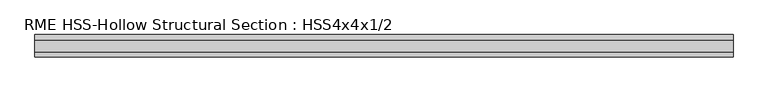
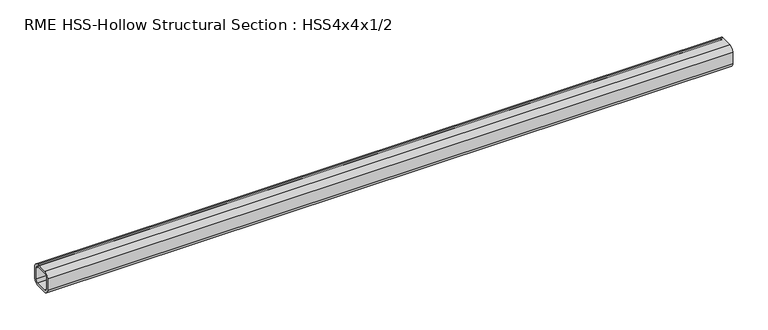
"""IFC4 building model written with IfcOpenShell, lengths in millimetres: member geometry, RME HSS-Hollow Structural Section : HSS4x4x1/2."""

import ifcopenshell
import ifcopenshell.guid

model = None  # the IFC model being written
_history = None  # IfcOwnerHistory: only IFC2X3 demands one
_inside = {}  # id of a spatial element -> (the spatial element, [elements in it])
_under = {}  # id of a project, library or spatial element -> (it, [spatial elements below it])
_declared = {}  # id of a project -> (the project, [libraries it declares])
_typed = {}  # id of a type object -> (the type object, [elements of that type])
_made_of = {}  # id of a material, layer set ... -> (it, [elements and type objects made of it])


def new_model(schema):
    """Start an empty IFC model of exactly this schema.

    Asked for "IFC4X3", IfcOpenShell would pick the latest addendum, in which some entities
    have other attributes; the version numbers below select the first issue.
    IFC2X3 requires an IfcOwnerHistory on every rooted entity: one is made here for all.
    """
    global model, _history
    if schema == "IFC4X3":
        model = ifcopenshell.file(schema_version=(4, 3, 0, 0))
    else:
        model = ifcopenshell.file(schema=schema)
    _inside.clear()
    _under.clear()
    _declared.clear()
    _typed.clear()
    _made_of.clear()
    _history = None
    if model.schema == "IFC2X3":
        org = make("IfcOrganization", Name="unknown")
        user = make(
            "IfcPersonAndOrganization",
            ThePerson=make("IfcPerson", FamilyName="unknown"),
            TheOrganization=org,
        )
        app = make(
            "IfcApplication",
            ApplicationDeveloper=org,
            Version="unknown",
            ApplicationFullName="unknown",
            ApplicationIdentifier="unknown",
        )
        _history = make(
            "IfcOwnerHistory",
            OwningUser=user,
            OwningApplication=app,
            ChangeAction="ADDED",
            CreationDate=0,
        )
    return model


def make(cls, **values):
    """One entity of the class cls with the attributes given. An attribute that is None is left unset."""
    return model.create_entity(
        cls, **{name: value for name, value in values.items() if value is not None}
    )


def rooted(cls, **values):
    """An entity with a GlobalId (a new one), such as an element, a storey or a relation."""
    return make(cls, GlobalId=ifcopenshell.guid.new(), OwnerHistory=_history, **values)


def si_unit(unit_type, name, prefix=None):
    """IfcSIUnit, for example si_unit("LENGTHUNIT", "METRE", prefix="MILLI")."""
    return make("IfcSIUnit", UnitType=unit_type, Prefix=prefix, Name=name)


def assignment(units):
    """IfcUnitAssignment: the units of a project."""
    return None if units is None else make("IfcUnitAssignment", Units=units)


def point(xyz):
    """IfcCartesianPoint."""
    return None if xyz is None else make("IfcCartesianPoint", Coordinates=xyz)


def direction(xyz):
    """IfcDirection."""
    return None if xyz is None else make("IfcDirection", DirectionRatios=xyz)


def frame(location, z_axis=None, x_axis=None):
    """IfcAxis2Placement3D, a coordinate frame: its origin and axes. An axis left out is left unset."""
    return make(
        "IfcAxis2Placement3D",
        Location=point(location),
        Axis=direction(z_axis),
        RefDirection=direction(x_axis),
    )


def frame_2d(location, x_axis=None):
    """IfcAxis2Placement2D, a coordinate frame in the plane: its origin and x axis."""
    return make(
        "IfcAxis2Placement2D", Location=point(location), RefDirection=direction(x_axis)
    )


def origin():
    """The frame at (0, 0, 0) with its axes left unset."""
    return frame((0.0, 0.0, 0.0))


def place(relative_to, where):
    """IfcLocalPlacement: puts the frame where relative to a parent placement (None: the world)."""
    return make(
        "IfcLocalPlacement", PlacementRelTo=relative_to, RelativePlacement=where
    )


def context(
    kind, dimensions, precision=None, world=None, true_north=None, identifier=None
):
    """IfcGeometricRepresentationContext, for example the 3D "Model" context."""
    return make(
        "IfcGeometricRepresentationContext",
        ContextIdentifier=identifier,
        ContextType=kind,
        CoordinateSpaceDimension=dimensions,
        Precision=precision,
        WorldCoordinateSystem=world,
        TrueNorth=true_north,
    )


def project(units=None, contexts=None):
    """IfcProject with its units and contexts."""
    return rooted(
        "IfcProject",
        Name="project",
        RepresentationContexts=contexts,
        UnitsInContext=assignment(units),
    )


def spatial(cls, under=None, at=None, **own):
    """A site, building, storey or space (cls), placed at a placement, below another one or the project."""
    s = rooted(cls, ObjectPlacement=at, **own)
    if under is not None:
        _under.setdefault(under.id(), (under, []))[1].append(s)
    return s


def polyline(points):
    """IfcPolyline through the points."""
    return make("IfcPolyline", Points=[point(p) for p in points])


def circle_curve(where, radius):
    """IfcCircle in the frame where."""
    return make("IfcCircle", Position=where, Radius=radius)


def trimmed(basis, trim1, trim2, sense, master):
    """IfcTrimmedCurve: the piece of a basis curve between two trims."""
    return make(
        "IfcTrimmedCurve",
        BasisCurve=basis,
        Trim1=trim1,
        Trim2=trim2,
        SenseAgreement=sense,
        MasterRepresentation=master,
    )


def segment(curve, same_sense, transition):
    """IfcCompositeCurveSegment."""
    return make(
        "IfcCompositeCurveSegment",
        Transition=transition,
        SameSense=same_sense,
        ParentCurve=curve,
    )


def composite_curve(segments, self_intersect=None):
    """IfcCompositeCurve: segments joined end to end."""
    return make("IfcCompositeCurve", Segments=segments, SelfIntersect=self_intersect)


def outline(outer, holes=None, kind="AREA"):
    """IfcArbitraryClosedProfileDef: a profile drawn as a closed curve; with holes, ...WithVoids."""
    if holes is None:
        return make("IfcArbitraryClosedProfileDef", ProfileType=kind, OuterCurve=outer)
    return make(
        "IfcArbitraryProfileDefWithVoids",
        ProfileType=kind,
        OuterCurve=outer,
        InnerCurves=holes,
    )


def extrude(swept, where, along, depth):
    """IfcExtrudedAreaSolid: the profile swept, set in the frame where, extruded along a direction by depth."""
    return make(
        "IfcExtrudedAreaSolid",
        SweptArea=swept,
        Position=where,
        ExtrudedDirection=direction(along),
        Depth=depth,
    )


def shape(context_of_items, identifier, shape_type, items):
    """IfcShapeRepresentation: the items that make up one representation, for example the "Body"."""
    return make(
        "IfcShapeRepresentation",
        ContextOfItems=context_of_items,
        RepresentationIdentifier=identifier,
        RepresentationType=shape_type,
        Items=items,
    )


def source(mapping_origin, context_of_items, identifier, shape_type, items):
    """IfcRepresentationMap: a shape defined once, which mapped items show again and again."""
    return make(
        "IfcRepresentationMap",
        MappingOrigin=mapping_origin,
        MappedRepresentation=shape(context_of_items, identifier, shape_type, items),
    )


def transform(
    local_origin,
    x_axis=None,
    y_axis=None,
    z_axis=None,
    scale=None,
    scale2=None,
    scale3=None,
    uniform=True,
):
    """IfcCartesianTransformationOperator3D, or its non-uniform kind. x_axis, y_axis, z_axis: its Axis1, 2, 3."""
    if uniform:
        return make(
            "IfcCartesianTransformationOperator3D",
            Axis1=direction(x_axis),
            Axis2=direction(y_axis),
            LocalOrigin=point(local_origin),
            Scale=scale,
            Axis3=direction(z_axis),
        )
    return make(
        "IfcCartesianTransformationOperator3DnonUniform",
        Axis1=direction(x_axis),
        Axis2=direction(y_axis),
        LocalOrigin=point(local_origin),
        Scale=scale,
        Axis3=direction(z_axis),
        Scale2=scale2,
        Scale3=scale3,
    )


def mapped(mapping_source, mapping_target):
    """IfcMappedItem: shows the shape of a source again, moved by a transform."""
    return make(
        "IfcMappedItem", MappingSource=mapping_source, MappingTarget=mapping_target
    )


def made_of(thing, what):
    """Note that an element or type object is made of a material, layer set ...; save() writes the relation."""
    if what is not None:
        _made_of.setdefault(what.id(), (what, []))[1].append(thing)
    return thing


def element(
    cls,
    number,
    at=None,
    inside=None,
    cuts=None,
    type_object=None,
    material=None,
    context=None,
    identifier="Body",
    shape_type=None,
    held_by="IfcProductDefinitionShape",
    body=None,
    shapes=None,
    **own,
):
    """One element of the class cls, such as IfcWall. Its Tag is "e" and its number.

    at: its placement. inside: the storey or other place that contains it. cuts: it is an
    opening in that element (IfcRelVoidsElement). A single representation is given by context,
    identifier, shape_type and body (its items); several are given by shapes. held_by: the class
    of the entity that holds the representations. save() writes the other relations.
    """
    e = rooted(cls, Tag="e%d" % number, ObjectPlacement=at, **own)
    if body is not None:
        shapes = [shape(context, identifier, shape_type, body)]
    if shapes is not None:
        e.Representation = make(held_by, Representations=shapes)
    if inside is not None:
        _inside.setdefault(inside.id(), (inside, []))[1].append(e)
    if cuts is not None:
        rooted(
            "IfcRelVoidsElement", RelatingBuildingElement=cuts, RelatedOpeningElement=e
        )
    if type_object is not None:
        _typed.setdefault(type_object.id(), (type_object, []))[1].append(e)
    return made_of(e, material)


def aggregate(whole, parts):
    """IfcRelAggregates: a whole, such as a stair, and the parts it consists of."""
    return rooted("IfcRelAggregates", RelatingObject=whole, RelatedObjects=parts)


def save(model, path):
    """Write the relations noted so far, then the file.

    IfcRelAggregates (storeys below a building ...), IfcRelContainedInSpatialStructure (elements
    in a storey), IfcRelDefinesByType, IfcRelAssociatesMaterial and IfcRelDeclares: one each for
    every whole, place, type object, material and project.
    """
    for whole, parts in _under.values():
        aggregate(whole, parts)
    for where, things in _inside.values():
        rooted(
            "IfcRelContainedInSpatialStructure",
            RelatedElements=things,
            RelatingStructure=where,
        )
    for kind, things in _typed.values():
        rooted("IfcRelDefinesByType", RelatedObjects=things, RelatingType=kind)
    for what, things in _made_of.values():
        rooted("IfcRelAssociatesMaterial", RelatedObjects=things, RelatingMaterial=what)
    for by, libraries in _declared.values():
        rooted("IfcRelDeclares", RelatingContext=by, RelatedDefinitions=libraries)
    model.write(path)


def rme_hss_hollow_structural_section_hss4x4x1_2_36c9f05c(model_context):
    return source(origin(), model_context, "Body", "SweptSolid", [
        extrude(outline(composite_curve([segment(polyline([(50.8, 27.178), (50.8, -27.178)]), True, "CONTINUOUS"), segment(trimmed(circle_curve(frame_2d((27.178, -27.178)), 23.622), [point((50.8, -27.178))], [point((27.178, -50.8))], False, "CARTESIAN"), True, "CONTINUOUS"), segment(polyline([(27.178, -50.8), (-27.178, -50.8)]), True, "CONTINUOUS"), segment(trimmed(circle_curve(frame_2d((-27.178, -27.178)), 23.622), [point((-27.178, -50.8))], [point((-50.8, -27.178))], False, "CARTESIAN"), True, "CONTINUOUS"), segment(polyline([(-50.8, -27.178), (-50.8, 27.178)]), True, "CONTINUOUS"), segment(trimmed(circle_curve(frame_2d((-27.178, 27.178)), 23.622), [point((-50.8, 27.178))], [point((-27.178, 50.8))], False, "CARTESIAN"), True, "CONTINUOUS"), segment(polyline([(-27.178, 50.8), (27.178, 50.8)]), True, "CONTINUOUS"), segment(trimmed(circle_curve(frame_2d((27.178, 27.178)), 23.622), [point((27.178, 50.8))], [point((50.8, 27.178))], False, "CARTESIAN"), True, "CONTINUOUS")], self_intersect=False), holes=[composite_curve([segment(trimmed(circle_curve(frame_2d((-27.178, 27.178)), 11.811), [point((-27.178, 38.989))], [point((-38.989, 27.178))], True, "CARTESIAN"), True, "CONTINUOUS"), segment(polyline([(-38.989, 27.178), (-38.989, -27.178)]), True, "CONTINUOUS"), segment(trimmed(circle_curve(frame_2d((-27.178, -27.178)), 11.811), [point((-38.989, -27.178))], [point((-27.178, -38.989))], True, "CARTESIAN"), True, "CONTINUOUS"), segment(polyline([(-27.178, -38.989), (27.178, -38.989)]), True, "CONTINUOUS"), segment(trimmed(circle_curve(frame_2d((27.178, -27.178)), 11.811), [point((27.178, -38.989))], [point((38.989, -27.178))], True, "CARTESIAN"), True, "CONTINUOUS"), segment(polyline([(38.989, -27.178), (38.989, 27.178)]), True, "CONTINUOUS"), segment(trimmed(circle_curve(frame_2d((27.178, 27.178)), 11.811), [point((38.989, 27.178))], [point((27.178, 38.989))], True, "CARTESIAN"), True, "CONTINUOUS"), segment(polyline([(27.178, 38.989), (-27.178, 38.989)]), True, "CONTINUOUS")], self_intersect=False)]), frame((-1483.4579653, 0.0, 0.0), z_axis=(1.0, 0.0, 0.0), x_axis=(0.0, 1.0, 0.0)), (0.0, 0.0, 1.0), 3149.7573153),
    ])


if __name__ == "__main__":
    model = new_model("IFC4")
    model_context = context("Model", 3, world=origin())
    ifc_project = project(units=[si_unit("LENGTHUNIT", "METRE", prefix="MILLI")], contexts=[model_context])
    site = spatial("IfcSite", under=ifc_project)
    building = spatial("IfcBuilding", under=site)
    placement = place(None, origin())
    rme_hss_hollow_structural_section_hss4x4x1_2_shape = rme_hss_hollow_structural_section_hss4x4x1_2_36c9f05c(model_context)
    element("IfcMember", 1, ObjectType="RME HSS-Hollow Structural Section : HSS4x4x1/2", at=placement, inside=building, context=model_context, shape_type="MappedRepresentation", body=[
        mapped(rme_hss_hollow_structural_section_hss4x4x1_2_shape, transform((0.0, 0.0, 0.0), x_axis=(1.0, 0.0, 0.0), y_axis=(0.0, 1.0, 0.0), z_axis=(0.0, 0.0, 1.0))),
    ])
    save(model, "model.ifc")

# Revit data of these elements
# Type "RME HSS-Hollow Structural Section : HSS4x4x1/2"
#   Nominal Size = "HSS6x4"
#   Assembly Code = "B10"
#   Shape = "Square"
#   W = 21.5
#   Start Extension Calculation [instance default] = 10' - 0"
#   Start Extension [instance default] = -0' - 0 1/2"
#   End Extension Calculation [instance default] = 10' - 0"
#   End Extension [instance default] = -0' - 0 1/2"
#   Ht = 0' - 4"
#   Length [instance default] = 5' - 0"
#   b = 0' - 4"
#   kr = 0' - 0.93"
#   t = 0' - 0.465"
#   A = 0.0418056 SF
#   Structural Material [instance default] = Metal - Steel - ASTM A500 - Grade B - Rectangular and Square
# Element 1 (IfcMember, "RME HSS-Hollow Structural Section : HSS4x4x1/2")
#   Length = 11' - 6.04926"
#   Structural Material = Metal - Steel - ASTM A992
#   Materials on its faces: "Metal - Steel - ASTM A992"
# Materials
#   "Metal - Steel - ASTM A500 - Grade B - Rectangular and Square": class "Metal", colour RGB 255 128 0, transparency 0
#   "Metal - Steel - ASTM A992": class "Metal", colour RGB 255 128 0, transparency 0
